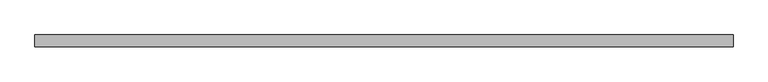
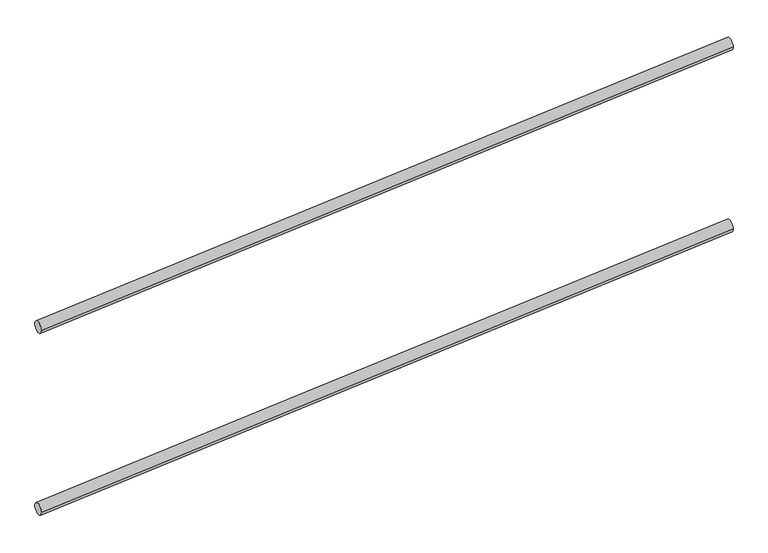
"""IFC4 building model written with IfcOpenShell, lengths in millimetres: railing geometry."""

from ifc_helpers import new_model, si_unit, frame, origin, place, context, project, spatial, ellipse_curve, source, transform, mapped, element, save
from ifc_brep_helpers import plane_surface, cylinder_surface, advanced_brep


def railing_fd78c9dc(model_context):
    return source(origin(), model_context, "Body", "AdvancedBrep", [
        advanced_brep(
        [(-2175.3, 16587.264479, 584.9480068), (-2175.3, 16617.264479, 584.9480068), (-375.3, 16587.264479, 734.9480068), (-375.3, 16617.264479, 734.9480068)],
        [
            (0, 1, ellipse_curve(frame((-2175.3, 16602.264479, 584.9480068), z_axis=(-1.0, 0.0, 0.0), x_axis=(0.0, 0.0, -0.9999999999999999)), 15.0519932, 15.0)),
            (1, 0, ellipse_curve(frame((-2175.3, 16602.264479, 584.9480068), z_axis=(-1.0, 0.0, 0.0), x_axis=(0.0, 0.0, -0.9999999999999999)), 15.0519932, 15.0)),
            (2, 3, ellipse_curve(frame((-375.3, 16602.264479, 734.9480068), z_axis=(1.0, 0.0, 0.0), x_axis=(0.0, 0.0, -0.9999999999999999)), 15.0519932, 15.0)),
            (3, 2, ellipse_curve(frame((-375.3, 16602.264479, 734.9480068), z_axis=(1.0, 0.0, 0.0), x_axis=(0.0, 0.0, -0.9999999999999999)), 15.0519932, 15.0)),
            (0, 2),
            (3, 1),
        ],
        [
            plane_surface(frame((-2175.3, 16602.264479, 600.0), z_axis=(-1.0, 0.0, 0.0), x_axis=(0.0, 1.0, 0.0))),
            plane_surface(frame((-375.3, 16602.264479, 750.0), z_axis=(1.0, 0.0, 0.0), x_axis=(0.0, 1.0, 0.0))),
            cylinder_surface(frame((-2174.0543178, 16602.264479, 585.0518136), z_axis=(-0.9965457582448797, 0.0, -0.08304547985373997), x_axis=(0.0, 1.0, 0.0)), 15.0),
        ],
        [
            (0, [[1, 2]]),
            (1, [[3, 4]]),
            (2, [[-1, 5, -4, 6]]),
            (2, [[-2, -6, -3, -5]]),
        ],
    ),
        advanced_brep(
        [(-2175.3, 16587.264479, 1084.9480068), (-2175.3, 16617.264479, 1084.9480068), (-375.3, 16587.264479, 1234.9480068), (-375.3, 16617.264479, 1234.9480068)],
        [
            (0, 1, ellipse_curve(frame((-2175.3, 16602.264479, 1084.9480068), z_axis=(-1.0, 0.0, 0.0), x_axis=(0.0, 0.0, -0.9999999999999999)), 15.0519932, 15.0)),
            (1, 0, ellipse_curve(frame((-2175.3, 16602.264479, 1084.9480068), z_axis=(-1.0, 0.0, 0.0), x_axis=(0.0, 0.0, -0.9999999999999999)), 15.0519932, 15.0)),
            (2, 3, ellipse_curve(frame((-375.3, 16602.264479, 1234.9480068), z_axis=(1.0, 0.0, 0.0), x_axis=(0.0, 0.0, -0.9999999999999999)), 15.0519932, 15.0)),
            (3, 2, ellipse_curve(frame((-375.3, 16602.264479, 1234.9480068), z_axis=(1.0, 0.0, 0.0), x_axis=(0.0, 0.0, -0.9999999999999999)), 15.0519932, 15.0)),
            (0, 2),
            (3, 1),
        ],
        [
            plane_surface(frame((-2175.3, 16602.264479, 1100.0), z_axis=(-1.0, 0.0, 0.0), x_axis=(0.0, 1.0, 0.0))),
            plane_surface(frame((-375.3, 16602.264479, 1250.0), z_axis=(1.0, 0.0, 0.0), x_axis=(0.0, 1.0, 0.0))),
            cylinder_surface(frame((-2174.0543178, 16602.264479, 1085.0518136), z_axis=(-0.9965457582448797, 0.0, -0.08304547985373997), x_axis=(0.0, 1.0, 0.0)), 15.0),
        ],
        [
            (0, [[1, 2]]),
            (1, [[3, 4]]),
            (2, [[-1, 5, -4, 6]]),
            (2, [[-2, -6, -3, -5]]),
        ],
    ),
    ])


if __name__ == "__main__":
    model = new_model("IFC4")
    model_context = context("Model", 3, world=origin())
    ifc_project = project(units=[si_unit("LENGTHUNIT", "METRE", prefix="MILLI")], contexts=[model_context])
    site = spatial("IfcSite", under=ifc_project)
    building = spatial("IfcBuilding", under=site)
    placement = place(None, origin())
    railing_shape = railing_fd78c9dc(model_context)
    element("IfcRailing", 1, at=placement, inside=building, context=model_context, shape_type="MappedRepresentation", body=[
        mapped(railing_shape, transform((0.0, 0.0, 0.0), x_axis=(1.0, 0.0, 0.0), y_axis=(0.0, 1.0, 0.0), z_axis=(0.0, 0.0, 1.0))),
    ])
    save(model, "model.ifc")
